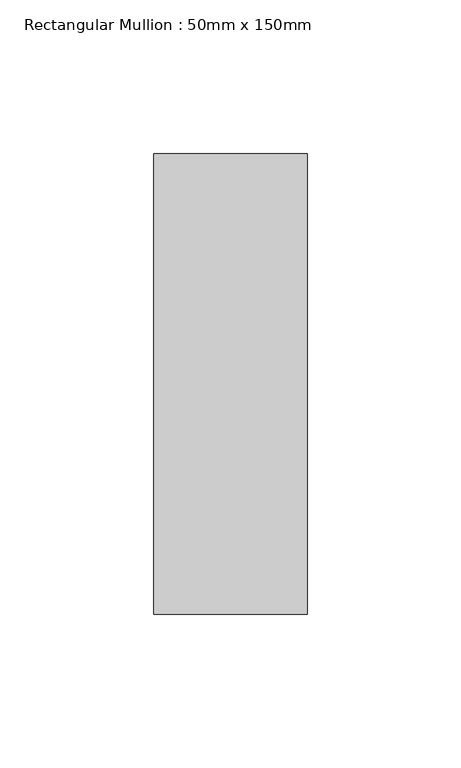
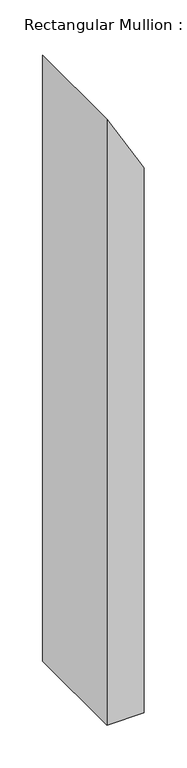
"""IFC4 building model written with IfcOpenShell, lengths in millimetres: member geometry, Rectangular Mullion : 50mm x 150mm."""

from ifc_helpers import new_model, si_unit, frame, origin, place, context, project, spatial, polyline, outline, extrude, source, transform, mapped, element, save


def rectangular_mullion_50mm_x_150mm_f9b92fbf(model_context):
    return source(origin(), model_context, "Body", "SweptSolid", [
        extrude(outline(polyline([(-143.3012702, 25.0), (-56.6987298, -25.0), (-918.1517015, -25.0), (-918.1517015, 25.0), (-143.3012702, 25.0)])), frame((0.0, -75.0, 0.0), z_axis=(0.0, 1.0, 0.0), x_axis=(0.0, 0.0, 1.0)), (0.0, 0.0, 1.0), 150.0),
    ])


if __name__ == "__main__":
    model = new_model("IFC4")
    model_context = context("Model", 3, world=origin())
    ifc_project = project(units=[si_unit("LENGTHUNIT", "METRE", prefix="MILLI")], contexts=[model_context])
    site = spatial("IfcSite", under=ifc_project)
    building = spatial("IfcBuilding", under=site)
    placement = place(None, origin())
    rectangular_mullion_50mm_x_150mm_shape = rectangular_mullion_50mm_x_150mm_f9b92fbf(model_context)
    element("IfcMember", 1, ObjectType="Rectangular Mullion : 50mm x 150mm", at=placement, inside=building, context=model_context, shape_type="MappedRepresentation", body=[
        mapped(rectangular_mullion_50mm_x_150mm_shape, transform((0.0, 0.0, 0.0), x_axis=(1.0, 0.0, 0.0), y_axis=(0.0, 1.0, 0.0), z_axis=(0.0, 0.0, 1.0))),
    ])
    save(model, "model.ifc")

# Revit data of these elements
# Type "Rectangular Mullion : 50mm x 150mm"
#   built-in parameter 1007304 = 0.492126 (stored number, unit not read)
#   built-in parameter 1007301 = 0.082021 (stored number, unit not read)
#   built-in parameter 1007300 = 0.082021 (stored number, unit not read)
# Element 1 (IfcMember, "Rectangular Mullion : 50mm x 150mm")
#   Materials on its faces: "Aluminum"
# Materials
#   "Aluminum": class "Metal", colour RGB 247 247 247, transparency 0, Description = "Aluminum 6061", Cost = 0
